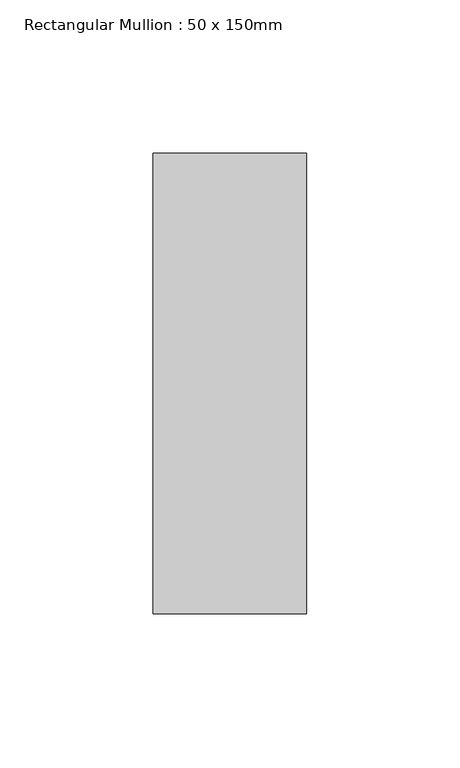
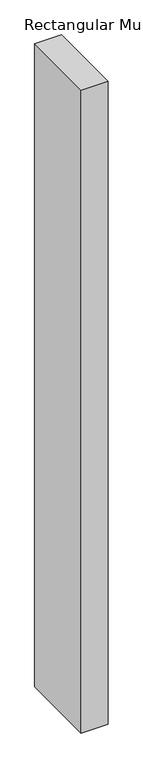
"""IFC4 building model written with IfcOpenShell, lengths in millimetres: member geometry, Rectangular Mullion : 50 x 150mm."""

from ifc_helpers import new_model, si_unit, frame, origin, place, context, project, spatial, polyline, outline, extrude, source, transform, mapped, element, save


def rectangular_mullion_50_x_150mm_97c2790d(model_context):
    return source(origin(), model_context, "Body", "SweptSolid", [
        extrude(outline(polyline([(25.0, 75.0), (25.0, -75.0), (-25.0, -75.0), (-25.0, 75.0), (25.0, 75.0)])), frame((0.0, 0.0, -1264.9999999), z_axis=(0.0, 0.0, 1.0), x_axis=(1.0, 0.0, 0.0)), (0.0, 0.0, 1.0), 1264.9999999),
    ])


if __name__ == "__main__":
    model = new_model("IFC4")
    model_context = context("Model", 3, world=origin())
    ifc_project = project(units=[si_unit("LENGTHUNIT", "METRE", prefix="MILLI")], contexts=[model_context])
    site = spatial("IfcSite", under=ifc_project)
    building = spatial("IfcBuilding", under=site)
    placement = place(None, origin())
    rectangular_mullion_50_x_150mm_shape = rectangular_mullion_50_x_150mm_97c2790d(model_context)
    element("IfcMember", 1, ObjectType="Rectangular Mullion : 50 x 150mm", at=placement, inside=building, context=model_context, shape_type="MappedRepresentation", body=[
        mapped(rectangular_mullion_50_x_150mm_shape, transform((0.0, 0.0, 0.0), x_axis=(1.0, 0.0, 0.0), y_axis=(0.0, 1.0, 0.0), z_axis=(0.0, 0.0, 1.0))),
    ])
    save(model, "model.ifc")

# Revit data of these elements
# Type "Rectangular Mullion : 50 x 150mm"
#   built-in parameter 1007304 = 0.492126 (stored number, unit not read)
#   built-in parameter 1007301 = 0.082021 (stored number, unit not read)
#   built-in parameter 1007300 = 0.082021 (stored number, unit not read)
# Element 1 (IfcMember, "Rectangular Mullion : 50 x 150mm")
#   Materials on its faces: "Aluminium"
# Materials
#   "Aluminium": class "Metal", colour RGB 247 247 247, transparency 0, Description = "Aluminium 6061", Cost = 0
